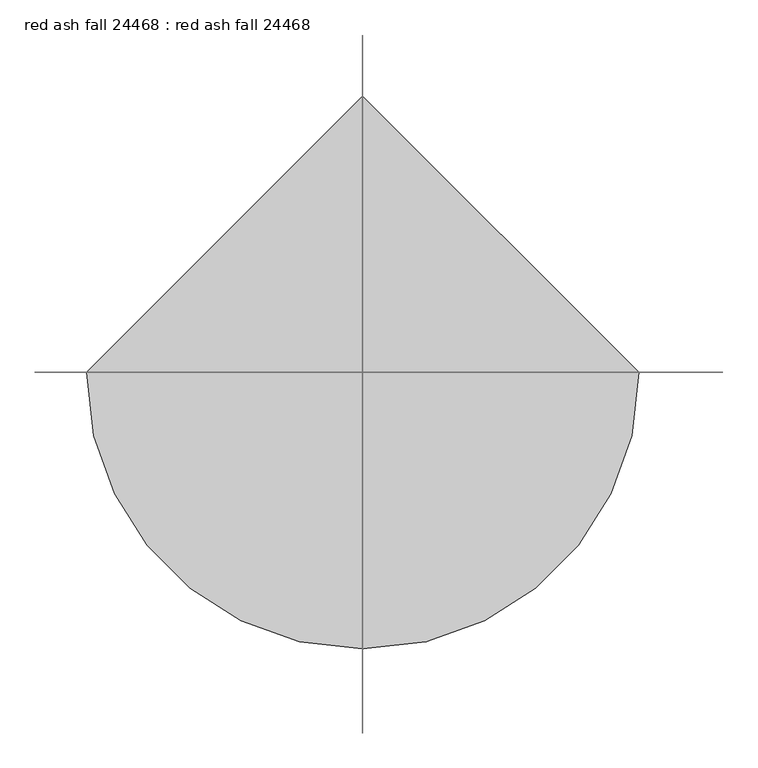
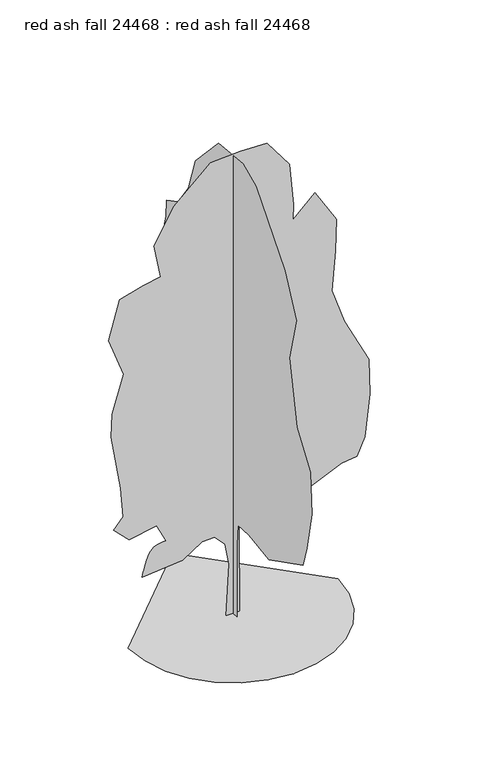
"""IFC4 building model written with IfcOpenShell, lengths in millimetres: proxy geometry, red ash fall 24468 : red ash fall 24468."""

import ifcopenshell
import ifcopenshell.guid

model = None  # the IFC model being written
_history = None  # IfcOwnerHistory: only IFC2X3 demands one
_inside = {}  # id of a spatial element -> (the spatial element, [elements in it])
_under = {}  # id of a project, library or spatial element -> (it, [spatial elements below it])
_declared = {}  # id of a project -> (the project, [libraries it declares])
_typed = {}  # id of a type object -> (the type object, [elements of that type])
_made_of = {}  # id of a material, layer set ... -> (it, [elements and type objects made of it])


def new_model(schema):
    """Start an empty IFC model of exactly this schema.

    Asked for "IFC4X3", IfcOpenShell would pick the latest addendum, in which some entities
    have other attributes; the version numbers below select the first issue.
    IFC2X3 requires an IfcOwnerHistory on every rooted entity: one is made here for all.
    """
    global model, _history
    if schema == "IFC4X3":
        model = ifcopenshell.file(schema_version=(4, 3, 0, 0))
    else:
        model = ifcopenshell.file(schema=schema)
    _inside.clear()
    _under.clear()
    _declared.clear()
    _typed.clear()
    _made_of.clear()
    _history = None
    if model.schema == "IFC2X3":
        org = make("IfcOrganization", Name="unknown")
        user = make(
            "IfcPersonAndOrganization",
            ThePerson=make("IfcPerson", FamilyName="unknown"),
            TheOrganization=org,
        )
        app = make(
            "IfcApplication",
            ApplicationDeveloper=org,
            Version="unknown",
            ApplicationFullName="unknown",
            ApplicationIdentifier="unknown",
        )
        _history = make(
            "IfcOwnerHistory",
            OwningUser=user,
            OwningApplication=app,
            ChangeAction="ADDED",
            CreationDate=0,
        )
    return model


def make(cls, **values):
    """One entity of the class cls with the attributes given. An attribute that is None is left unset."""
    return model.create_entity(
        cls, **{name: value for name, value in values.items() if value is not None}
    )


def rooted(cls, **values):
    """An entity with a GlobalId (a new one), such as an element, a storey or a relation."""
    return make(cls, GlobalId=ifcopenshell.guid.new(), OwnerHistory=_history, **values)


def si_unit(unit_type, name, prefix=None):
    """IfcSIUnit, for example si_unit("LENGTHUNIT", "METRE", prefix="MILLI")."""
    return make("IfcSIUnit", UnitType=unit_type, Prefix=prefix, Name=name)


def assignment(units):
    """IfcUnitAssignment: the units of a project."""
    return None if units is None else make("IfcUnitAssignment", Units=units)


def point(xyz):
    """IfcCartesianPoint."""
    return None if xyz is None else make("IfcCartesianPoint", Coordinates=xyz)


def direction(xyz):
    """IfcDirection."""
    return None if xyz is None else make("IfcDirection", DirectionRatios=xyz)


def frame(location, z_axis=None, x_axis=None):
    """IfcAxis2Placement3D, a coordinate frame: its origin and axes. An axis left out is left unset."""
    return make(
        "IfcAxis2Placement3D",
        Location=point(location),
        Axis=direction(z_axis),
        RefDirection=direction(x_axis),
    )


def origin():
    """The frame at (0, 0, 0) with its axes left unset."""
    return frame((0.0, 0.0, 0.0))


def place(relative_to, where):
    """IfcLocalPlacement: puts the frame where relative to a parent placement (None: the world)."""
    return make(
        "IfcLocalPlacement", PlacementRelTo=relative_to, RelativePlacement=where
    )


def context(
    kind, dimensions, precision=None, world=None, true_north=None, identifier=None
):
    """IfcGeometricRepresentationContext, for example the 3D "Model" context."""
    return make(
        "IfcGeometricRepresentationContext",
        ContextIdentifier=identifier,
        ContextType=kind,
        CoordinateSpaceDimension=dimensions,
        Precision=precision,
        WorldCoordinateSystem=world,
        TrueNorth=true_north,
    )


def project(units=None, contexts=None):
    """IfcProject with its units and contexts."""
    return rooted(
        "IfcProject",
        Name="project",
        RepresentationContexts=contexts,
        UnitsInContext=assignment(units),
    )


def spatial(cls, under=None, at=None, **own):
    """A site, building, storey or space (cls), placed at a placement, below another one or the project."""
    s = rooted(cls, ObjectPlacement=at, **own)
    if under is not None:
        _under.setdefault(under.id(), (under, []))[1].append(s)
    return s


def point_list(points):
    """IfcCartesianPointList2D or 3D."""
    cls = (
        "IfcCartesianPointList2D" if len(points[0]) == 2 else "IfcCartesianPointList3D"
    )
    return make(cls, CoordList=points)


def triangles(points, corners, closed=None, point_numbers=None):
    """IfcTriangulatedFaceSet: each triangle names its three corners, points numbered from 1."""
    return make(
        "IfcTriangulatedFaceSet",
        Coordinates=point_list(points),
        Closed=closed,
        CoordIndex=corners,
        PnIndex=point_numbers,
    )


def shape(context_of_items, identifier, shape_type, items):
    """IfcShapeRepresentation: the items that make up one representation, for example the "Body"."""
    return make(
        "IfcShapeRepresentation",
        ContextOfItems=context_of_items,
        RepresentationIdentifier=identifier,
        RepresentationType=shape_type,
        Items=items,
    )


def source(mapping_origin, context_of_items, identifier, shape_type, items):
    """IfcRepresentationMap: a shape defined once, which mapped items show again and again."""
    return make(
        "IfcRepresentationMap",
        MappingOrigin=mapping_origin,
        MappedRepresentation=shape(context_of_items, identifier, shape_type, items),
    )


def transform(
    local_origin,
    x_axis=None,
    y_axis=None,
    z_axis=None,
    scale=None,
    scale2=None,
    scale3=None,
    uniform=True,
):
    """IfcCartesianTransformationOperator3D, or its non-uniform kind. x_axis, y_axis, z_axis: its Axis1, 2, 3."""
    if uniform:
        return make(
            "IfcCartesianTransformationOperator3D",
            Axis1=direction(x_axis),
            Axis2=direction(y_axis),
            LocalOrigin=point(local_origin),
            Scale=scale,
            Axis3=direction(z_axis),
        )
    return make(
        "IfcCartesianTransformationOperator3DnonUniform",
        Axis1=direction(x_axis),
        Axis2=direction(y_axis),
        LocalOrigin=point(local_origin),
        Scale=scale,
        Axis3=direction(z_axis),
        Scale2=scale2,
        Scale3=scale3,
    )


def mapped(mapping_source, mapping_target):
    """IfcMappedItem: shows the shape of a source again, moved by a transform."""
    return make(
        "IfcMappedItem", MappingSource=mapping_source, MappingTarget=mapping_target
    )


def made_of(thing, what):
    """Note that an element or type object is made of a material, layer set ...; save() writes the relation."""
    if what is not None:
        _made_of.setdefault(what.id(), (what, []))[1].append(thing)
    return thing


def element(
    cls,
    number,
    at=None,
    inside=None,
    cuts=None,
    type_object=None,
    material=None,
    context=None,
    identifier="Body",
    shape_type=None,
    held_by="IfcProductDefinitionShape",
    body=None,
    shapes=None,
    **own,
):
    """One element of the class cls, such as IfcWall. Its Tag is "e" and its number.

    at: its placement. inside: the storey or other place that contains it. cuts: it is an
    opening in that element (IfcRelVoidsElement). A single representation is given by context,
    identifier, shape_type and body (its items); several are given by shapes. held_by: the class
    of the entity that holds the representations. save() writes the other relations.
    """
    e = rooted(cls, Tag="e%d" % number, ObjectPlacement=at, **own)
    if body is not None:
        shapes = [shape(context, identifier, shape_type, body)]
    if shapes is not None:
        e.Representation = make(held_by, Representations=shapes)
    if inside is not None:
        _inside.setdefault(inside.id(), (inside, []))[1].append(e)
    if cuts is not None:
        rooted(
            "IfcRelVoidsElement", RelatingBuildingElement=cuts, RelatedOpeningElement=e
        )
    if type_object is not None:
        _typed.setdefault(type_object.id(), (type_object, []))[1].append(e)
    return made_of(e, material)


def aggregate(whole, parts):
    """IfcRelAggregates: a whole, such as a stair, and the parts it consists of."""
    return rooted("IfcRelAggregates", RelatingObject=whole, RelatedObjects=parts)


def save(model, path):
    """Write the relations noted so far, then the file.

    IfcRelAggregates (storeys below a building ...), IfcRelContainedInSpatialStructure (elements
    in a storey), IfcRelDefinesByType, IfcRelAssociatesMaterial and IfcRelDeclares: one each for
    every whole, place, type object, material and project.
    """
    for whole, parts in _under.values():
        aggregate(whole, parts)
    for where, things in _inside.values():
        rooted(
            "IfcRelContainedInSpatialStructure",
            RelatedElements=things,
            RelatingStructure=where,
        )
    for kind, things in _typed.values():
        rooted("IfcRelDefinesByType", RelatedObjects=things, RelatingType=kind)
    for what, things in _made_of.values():
        rooted("IfcRelAssociatesMaterial", RelatedObjects=things, RelatingMaterial=what)
    for by, libraries in _declared.values():
        rooted("IfcRelDeclares", RelatingContext=by, RelatedDefinitions=libraries)
    model.write(path)


def red_ash_fall_24468_red_ash_fall_24468_841d54ac(model_context):
    return source(origin(), model_context, "Body", "Tessellation", [
        triangles([(-1644.9506115, 0.0, 6.19e-05), (-1601.463295, -376.9127495, 6.19e-05), (-1477.6130058, -723.0483805, 6.19e-05), (-1283.3159992, -1028.488167, 6.19e-05), (-1028.488167, -1283.3159992, 6.19e-05), (-723.0483805, -1477.6130058, 6.19e-05), (-376.9127495, -1601.463295, 6.19e-05), (7.19e-05, -1644.9506115, 6.19e-05), (376.9127495, -1601.463295, 6.19e-05), (723.0483805, -1477.6130058, 6.19e-05), (1028.488167, -1283.3159992, 6.19e-05), (1283.3159992, -1028.488167, 6.19e-05), (1477.6130058, -723.0483805, 6.19e-05), (1601.463295, -376.9127495, 6.19e-05), (1644.9506115, 0.0001438, 6.19e-05), (-0.0002157, 1644.9506115, 6.19e-05), (-1.07e-05, -102.8462751, 0.0), (2.5e-05, -101.2465816, 1194.5531759), (3.23e-05, -129.8817524, 1537.8007565), (7e-07, -438.8252131, 1558.1640484), (-5.78e-05, -976.3902569, 1478.3064228), (-0.0001405, -1903.6900509, 1948.6758224), (-0.0001413, -2011.2029652, 2298.0931572), (-0.0001361, -2145.594326, 2943.1712242), (-0.0001119, -2105.2794903, 3615.1275925), (-5.81e-05, -1740.3808331, 4141.0085747), (-5.5e-06, -1527.397031, 5160.6396515), (-3.5e-06, -1715.5422329, 5886.3424484), (4.79e-05, -1406.4448208, 6531.4257477), (0.0001569, -626.9729948, 7458.7278671), (0.0001985, -273.1995851, 7618.189064), (0.0002662, 394.4006355, 7552.8093338), (0.0003121, 1026.0396246, 6880.8276764), (0.0003149, 1214.1899134, 6316.3894547), (0.0003323, 1496.4089516, 5913.2158081), (0.0003598, 1805.5114506, 5751.9512329), (0.0003531, 1818.9506012, 5483.1688019), (0.0003523, 1899.5853596, 5174.076622), (0.0003275, 1765.1941441, 4811.2124336), (0.0003297, 1886.146209, 4461.7849251), (0.0003279, 2007.0984192, 3977.9914902), (0.0003211, 1980.220118, 3843.6002747), (0.0002877, 1751.7549934, 3521.0461258), (0.0002729, 1737.3099449, 3077.5624397), (0.0002632, 1724.8766922, 2795.3433289), (0.0002542, 1738.3158428, 2445.9236687), (0.0002412, 1751.7549934, 1962.1149731), (0.0002172, 1563.6071754, 1814.2846069), (0.0001807, 1214.1899134, 1814.2846069), (0.0001827, 1375.4593575, 1317.0369061), (0.0001715, 1348.4948696, 1034.8838522), (0.0001516, 1103.0294746, 1227.8347927), (9.86e-05, 629.4621597, 1106.7073751), (9.8e-05, 551.7102922, 1357.0597538), (6.29e-05, 215.912475, 1354.0015102), (5.03e-05, 130.8009823, 1228.3325821), (3.27e-05, 79.5491688, 818.2830471), (1.17e-05, 112.1657825, 1.28e-05), (-110.8706308, 4.8e-06, 4.46e-05), (-66.7115076, -9.64e-05, 833.5001415), (-129.3072053, -0.000136, 1187.9415882), (-290.7865203, -0.00015, 1365.317244), (-483.63585, -0.0001408, 1358.6954098), (-796.2663677, -0.000103, 1155.7673893), (-1427.9079002, -6.9e-05, 1102.0109322), (-1419.1702068, -7.35e-05, 1136.7631714), (-1409.8433052, -7.82e-05, 1172.6914289), (-1399.343074, -8.32e-05, 1210.9717232), (-1387.0798691, -8.87e-05, 1252.7800724), (-1372.4647728, -9.49e-05, 1299.2874081), (-1354.9133732, -0.0001019, 1351.6722919), (-1333.8339912, -0.0001099, 1411.110815), (-1307.2681709, -0.0001176, 1466.2389908), (-1274.3547729, -0.0001239, 1506.5562973), (-1236.1533257, -0.0001289, 1534.5292992), (-1193.7200872, -0.0001329, 1552.6318279), (-1148.1144407, -0.0001362, 1563.327832), (-1100.3903915, -0.000139, 1569.0885269), (-1051.6097208, -0.0001415, 1572.3803318), (-1199.4401596, -0.0001703, 1868.0410641), (-1629.4947235, -0.0001418, 1787.4063057), (-1871.3989986, -0.0001601, 2029.3105808), (-1723.5686325, -0.0001874, 2204.0192482), (-1763.8834682, -0.0002433, 2687.8251823), (-1911.7164505, -0.0003442, 3588.2545235), (-1898.477869, -0.0003892, 3961.1515297), (-1719.9160938, -0.0004688, 4563.30867), (-1952.033757, -0.0005347, 5200.9494003), (-1777.3226189, -0.000616, 5819.1593399), (-1414.4661335, -0.0006447, 5926.6521973), (-1138.4116173, -0.0006626, 5975.3439926), (-1239.7574661, -0.0007228, 6517.9893585), (-930.6575832, -0.000802, 7068.9906097), (-352.7751603, -0.0008897, 7593.1190826), (117.5945209, -0.0009135, 7619.9924423), (534.2071818, -0.0009301, 7606.5560532), (883.6270237, -0.0008893, 7136.1737183), (947.8711401, -0.00081, 6447.504126), (938.6459038, -0.0007795, 6194.9520996), (1286.8008156, -0.0008333, 6517.9893585), (1622.7789997, -0.0007823, 5966.9875259), (1609.3398491, -0.0007196, 5446.5163879), (1549.4568764, -0.00064, 4800.6459274), (1743.7310646, -0.0005809, 4233.337532), (2131.7614494, -0.0005067, 3469.2048134), (2144.1338047, -0.0004386, 2892.8030777), (2066.2700981, -0.0003531, 2204.0192482), (1945.3180332, -0.0003141, 1921.7976665), (1703.4137581, -0.0003003, 1894.9193653), (1233.0443584, -0.0002542, 1679.8933914), (816.4288725, -0.0002007, 1384.2325138), (257.4769983, -0.0002049, 1624.5671173), (93.0507792, -0.0001766, 1447.6334404), (104.1551341, -4.6e-06, 3.52e-05)], [[15, 16, 1], [14, 15, 1], [14, 1, 2], [13, 14, 2], [13, 2, 3], [13, 3, 4], [12, 13, 4], [11, 12, 4], [11, 4, 5], [11, 5, 6], [11, 6, 7], [11, 7, 8], [11, 8, 9], [11, 9, 10], [50, 51, 52], [57, 58, 17], [57, 17, 18], [56, 57, 18], [56, 18, 19], [55, 56, 19], [49, 50, 52], [52, 53, 54], [49, 52, 54], [35, 36, 37], [46, 47, 48], [46, 48, 49], [21, 22, 23], [20, 21, 23], [20, 23, 24], [20, 24, 25], [20, 25, 26], [19, 20, 26], [19, 26, 27], [45, 46, 49], [31, 32, 33], [30, 31, 33], [29, 30, 33], [29, 33, 34], [28, 29, 34], [27, 28, 34], [19, 27, 34], [19, 34, 35], [19, 35, 37], [19, 37, 38], [19, 38, 39], [19, 39, 40], [19, 40, 41], [19, 41, 42], [19, 42, 43], [19, 43, 44], [19, 44, 45], [19, 45, 49], [19, 49, 54], [55, 19, 54], [64, 65, 66], [64, 66, 67], [64, 67, 68], [99, 100, 101], [64, 68, 69], [64, 69, 70], [64, 70, 71], [114, 59, 60], [113, 114, 60], [113, 60, 61], [113, 61, 62], [64, 71, 72], [64, 72, 73], [64, 73, 74], [64, 74, 75], [64, 75, 76], [64, 76, 77], [64, 77, 78], [64, 78, 79], [63, 64, 79], [81, 82, 83], [80, 81, 83], [99, 101, 102], [107, 108, 109], [110, 111, 112], [88, 89, 90], [87, 88, 90], [87, 90, 91], [80, 83, 84], [95, 96, 97], [95, 97, 98], [94, 95, 98], [93, 94, 98], [92, 93, 98], [91, 92, 98], [91, 98, 99], [87, 91, 99], [87, 99, 102], [87, 102, 103], [87, 103, 104], [86, 87, 104], [85, 86, 104], [84, 85, 104], [80, 84, 104], [80, 104, 105], [80, 105, 106], [80, 106, 107], [80, 107, 109], [80, 109, 110], [80, 110, 112], [79, 80, 112], [63, 79, 112], [62, 63, 112], [113, 62, 112]], closed=False),
    ])


if __name__ == "__main__":
    model = new_model("IFC4")
    model_context = context("Model", 3, world=origin())
    ifc_project = project(units=[si_unit("LENGTHUNIT", "METRE", prefix="MILLI")], contexts=[model_context])
    site = spatial("IfcSite", under=ifc_project)
    building = spatial("IfcBuilding", under=site)
    placement = place(None, origin())
    red_ash_fall_24468_red_ash_fall_24468_shape = red_ash_fall_24468_red_ash_fall_24468_841d54ac(model_context)
    element("IfcBuildingElementProxy", 1, Name="red ash fall 24468 : red ash fall 24468", ObjectType="red ash fall 24468 : red ash fall 24468", at=placement, inside=building, context=model_context, shape_type="MappedRepresentation", body=[
        mapped(red_ash_fall_24468_red_ash_fall_24468_shape, transform((0.0, 0.0, 0.0), x_axis=(1.0, 0.0, 0.0), y_axis=(0.0, 1.0, 0.0), z_axis=(0.0, 0.0, 1.0))),
    ])
    save(model, "model.ifc")

# Revit data of these elements
# Type "red ash fall 24468 : red ash fall 24468"
#   built-in parameter 1005195 = "RPC-16-G3AB-Q57X-UE54-U000-ST1L-LVER-AU"
#   Height = 0
